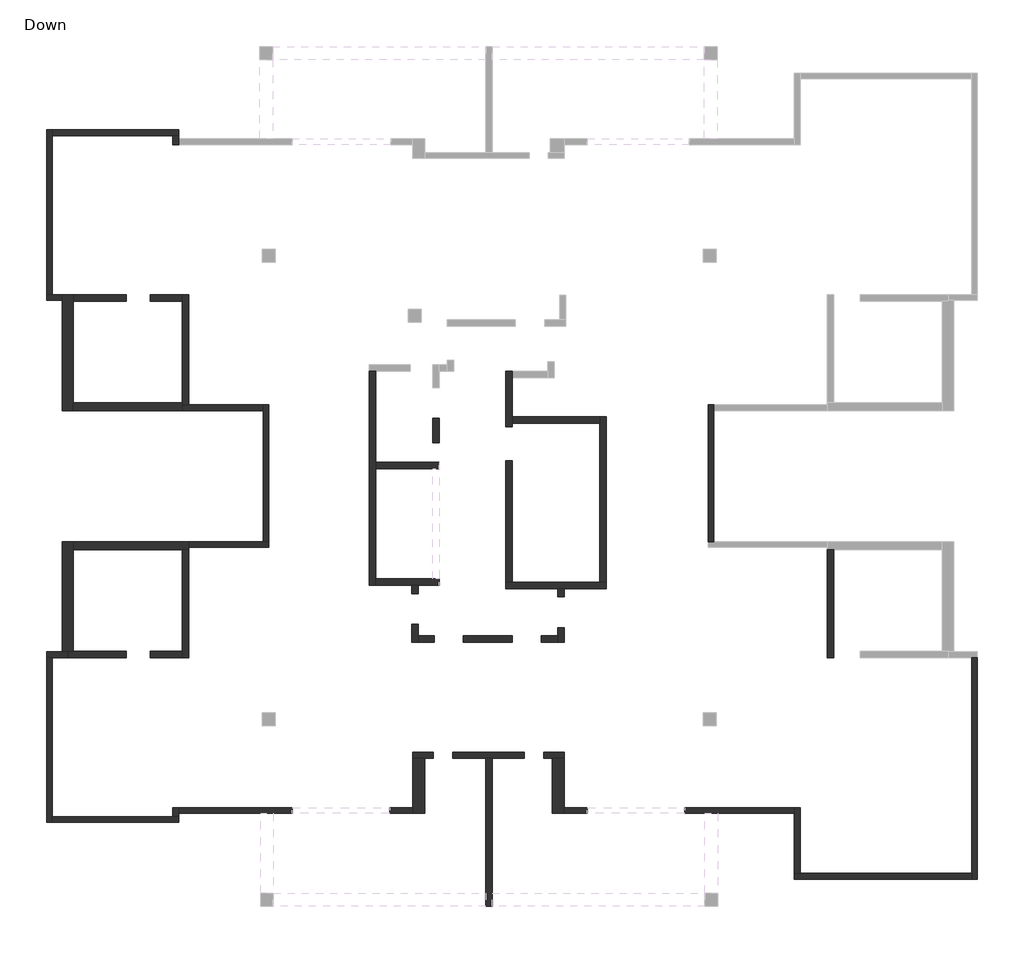
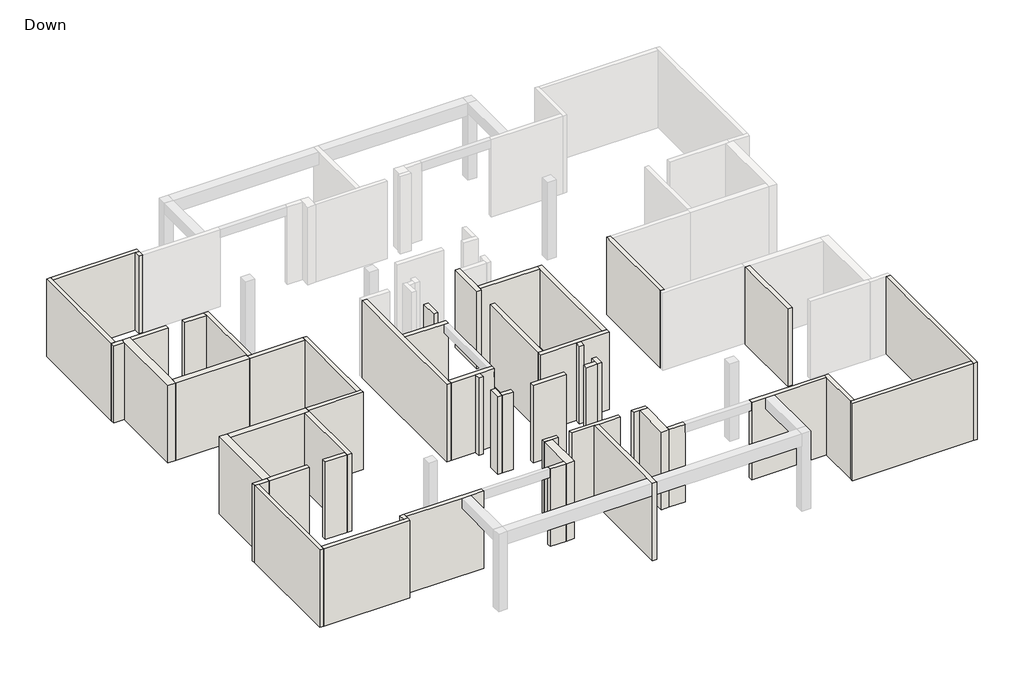
# One storey, part 1 of 2: 52 walls.
"""IFC4 building model written with IfcOpenShell, lengths in millimetres."""

from ifc_helpers import new_model, si_unit, origin, place, context, project, spatial, faceted_brep, element, save

model = new_model("IFC4")

# Units and contexts
model_context = context("Model", 3, world=origin())
ifc_project = project(units=[si_unit("LENGTHUNIT", "METRE", prefix="MILLI")], contexts=[model_context])

# Site, building, storey
site = spatial("IfcSite", under=ifc_project)
building = spatial("IfcBuilding", under=site)
storey = spatial("IfcBuildingStorey", under=building, Name="Down", Elevation=0.0)

# Walls
placement = place(None, origin())
element("IfcWall", 1, ObjectType="18", at=placement, inside=storey, context=model_context, shape_type="Brep", body=[
    faceted_brep([(-36860.6830632, 7917.598694, 0.0), (-36860.6830632, 2837.5734489, 0.0), (-36860.6830632, 2837.5734489, 3700.0), (-36860.6830632, 7917.598694, 3700.0), (-36680.6830632, 7917.598694, 0.0), (-36680.6830632, 7917.598694, 3540.0), (-36680.6830632, 7917.598694, 3700.0), (-36680.6830632, 3017.5734489, 3700.0), (-36680.6830632, 2837.5734489, 3700.0), (-36680.6830632, 2837.5734489, 0.0), (-36680.6830632, 3017.5734489, 0.0)], [[[0, 1, 2, 3]], [[4, 5, 6, 7, 8, 9, 10]], [[1, 0, 4, 10, 9]], [[3, 2, 8, 7, 6]], [[2, 1, 9, 8]], [[0, 3, 6, 5, 4]]]),
])
element("IfcWall", 2, ObjectType="18", at=placement, inside=storey, context=model_context, shape_type="Brep", body=[
    faceted_brep([(-36680.6830632, 2837.5734489, 0.0), (-32781.782199, 2837.5734489, 0.0), (-32781.782199, 2837.5734489, 3700.0), (-36680.6830632, 2837.5734489, 3700.0), (-36680.6830632, 3017.5734489, 0.0), (-36680.6830632, 3017.5734489, 3540.0), (-36680.6830632, 3017.5734489, 3700.0), (-32961.782199, 3017.5734489, 3700.0), (-32781.782199, 3017.5734489, 3700.0), (-32781.782199, 3017.5734489, 0.0), (-32961.782199, 3017.5734489, 0.0)], [[[0, 1, 2, 3]], [[4, 5, 6, 7, 8, 9, 10]], [[1, 0, 4, 10, 9]], [[3, 2, 8, 7, 6]], [[0, 3, 6, 5, 4]], [[2, 1, 9, 8]]]),
])
element("IfcWall", 3, ObjectType="18", at=placement, inside=storey, context=model_context, shape_type="Brep", body=[
    faceted_brep([(-32781.782199, 3017.5734489, 0.0), (-32781.782199, 3116.899597, 0.0), (-32781.782199, 3296.899597, 0.0), (-32781.782199, 3296.899597, 3700.0), (-32781.782199, 3116.899597, 3700.0), (-32781.782199, 3017.5734489, 3700.0), (-32961.782199, 3017.5734489, 0.0), (-32961.782199, 3017.5734489, 3540.0), (-32961.782199, 3017.5734489, 3700.0), (-32961.782199, 3296.899597, 3700.0), (-32961.782199, 3296.899597, 3540.0), (-32961.782199, 3296.899597, 0.0)], [[[0, 1, 2, 3, 4, 5]], [[6, 7, 8, 9, 10, 11]], [[2, 1, 0, 6, 11]], [[5, 4, 3, 9, 8]], [[0, 5, 8, 7, 6]], [[3, 2, 11, 10, 9]]]),
])
element("IfcWall", 4, ObjectType="18", at=placement, inside=storey, context=model_context, shape_type="Brep", body=[
    faceted_brep([(-32781.782199, 3116.899597, 0.0), (-29280.7432632, 3116.899597, 0.0), (-29280.7432632, 3116.899597, 3300.0), (-29280.7432632, 3116.899597, 3700.0), (-29861.4923547, 3116.899597, 3700.0), (-30261.4923547, 3116.899597, 3700.0), (-32781.782199, 3116.899597, 3700.0), (-32781.782199, 3296.899597, 0.0), (-32781.782199, 3296.899597, 3700.0), (-29280.7432632, 3296.899597, 3700.0), (-29280.7432632, 3296.899597, 3300.0), (-29280.7432632, 3296.899597, 0.0)], [[[0, 1, 2, 3, 4, 5, 6]], [[7, 8, 9, 10, 11]], [[1, 0, 7, 11]], [[3, 2, 1, 11, 10, 9]], [[6, 5, 4, 3, 9, 8]], [[0, 6, 8, 7]]]),
])
element("IfcWall", 5, ObjectType="18", at=placement, inside=storey, context=model_context, shape_type="Brep", body=[
    faceted_brep([(-26281.3646827, 3116.899597, 0.0), (-25559.7256887, 3116.899597, 0.0), (-25559.7256887, 3116.899597, 3700.0), (-26281.3646827, 3116.899597, 3700.0), (-26281.3646827, 3116.899597, 3300.0), (-26281.3646827, 3296.899597, 0.0), (-26281.3646827, 3296.899597, 3300.0), (-26281.3646827, 3296.899597, 3700.0), (-25559.7256887, 3296.899597, 3700.0), (-25559.7256887, 3296.899597, 3540.0), (-25559.7256887, 3296.899597, 0.0)], [[[0, 1, 2, 3, 4]], [[5, 6, 7, 8, 9, 10]], [[1, 0, 5, 10]], [[3, 2, 8, 7]], [[0, 4, 3, 7, 6, 5]], [[2, 1, 10, 9, 8]]]),
])
element("IfcWall", 6, ObjectType="18", at=placement, inside=storey, context=model_context, shape_type="Brep", body=[
    faceted_brep([(-25559.7256887, 4816.6180163, 0.0), (-25199.7256887, 4816.6180163, 0.0), (-24930.9034729, 4816.6180163, 0.0), (-24930.9034729, 4816.6180163, 3540.0), (-24930.9034729, 4816.6180163, 3700.0), (-25199.7256887, 4816.6180163, 3700.0), (-25559.7256887, 4816.6180163, 3700.0), (-25559.7256887, 4996.6180163, 0.0), (-25559.7256887, 4996.6180163, 3540.0), (-25559.7256887, 4996.6180163, 3700.0), (-24930.9034729, 4996.6180163, 3700.0), (-24930.9034729, 4996.6180163, 3540.0), (-24930.9034729, 4996.6180163, 0.0)], [[[0, 1, 2, 3, 4, 5, 6]], [[7, 8, 9, 10, 11, 12]], [[2, 1, 0, 7, 12]], [[4, 3, 2, 12, 11, 10]], [[6, 5, 4, 10, 9]], [[0, 6, 9, 8, 7]]]),
])
element("IfcWall", 7, ObjectType="18", at=placement, inside=storey, context=model_context, shape_type="Brep", body=[
    faceted_brep([(-24329.7577306, 4816.6180163, 0.0), (-23311.6200473, 4816.6180163, 0.0), (-23111.6200473, 4816.6180163, 0.0), (-22130.4956663, 4816.6180163, 0.0), (-22130.4956663, 4816.6180163, 3540.0), (-22130.4956663, 4816.6180163, 3700.0), (-23111.6200473, 4816.6180163, 3700.0), (-23311.6200473, 4816.6180163, 3700.0), (-24329.7577306, 4816.6180163, 3700.0), (-24329.7577306, 4816.6180163, 3540.0), (-24329.7577306, 4996.6180163, 0.0), (-24329.7577306, 4996.6180163, 3540.0), (-24329.7577306, 4996.6180163, 3700.0), (-22130.4956663, 4996.6180163, 3700.0), (-22130.4956663, 4996.6180163, 3540.0), (-22130.4956663, 4996.6180163, 0.0)], [[[0, 1, 2, 3, 4, 5, 6, 7, 8, 9]], [[10, 11, 12, 13, 14, 15]], [[3, 2, 1, 0, 10, 15]], [[5, 4, 3, 15, 14, 13]], [[8, 7, 6, 5, 13, 12]], [[0, 9, 8, 12, 11, 10]]]),
])
element("IfcWall", 8, ObjectType="18", at=placement, inside=storey, context=model_context, shape_type="Brep", body=[
    faceted_brep([(-36860.6830632, 7917.598694, 0.0), (-36680.6830632, 7917.598694, 0.0), (-36205.9326019, 7917.598694, 0.0), (-36205.9326019, 7917.598694, 3540.0), (-36205.9326019, 7917.598694, 3700.0), (-36680.6830632, 7917.598694, 3700.0), (-36860.6830632, 7917.598694, 3700.0), (-36860.6830632, 8097.598694, 0.0), (-36860.6830632, 8097.598694, 3700.0), (-36380.9326019, 8097.598694, 3700.0), (-36205.9326019, 8097.598694, 3700.0), (-36205.9326019, 8097.598694, 0.0), (-36380.9326019, 8097.598694, 0.0)], [[[0, 1, 2, 3, 4, 5, 6]], [[7, 8, 9, 10, 11, 12]], [[2, 1, 0, 7, 12, 11]], [[4, 3, 2, 11, 10]], [[6, 5, 4, 10, 9, 8]], [[0, 6, 8, 7]]]),
])
element("IfcWall", 9, ObjectType="18", at=placement, inside=storey, context=model_context, shape_type="Brep", body=[
    faceted_brep([(-32480.1801017, 11317.0355326, 0.0), (-30000.4247857, 11317.0355326, 0.0), (-30000.4247857, 11317.0355326, 3540.0), (-30000.4247857, 11317.0355326, 3700.0), (-32480.1801017, 11317.0355326, 3700.0), (-32480.1801017, 11317.0355326, 3540.0), (-32480.1801017, 11497.0355326, 0.0), (-32480.1801017, 11497.0355326, 3700.0), (-30180.4247857, 11497.0355326, 3700.0), (-30000.4247857, 11497.0355326, 3700.0), (-30000.4247857, 11497.0355326, 0.0), (-30180.4247857, 11497.0355326, 0.0)], [[[0, 1, 2, 3, 4, 5]], [[6, 7, 8, 9, 10, 11]], [[1, 0, 6, 11, 10]], [[4, 3, 9, 8, 7]], [[0, 5, 4, 7, 6]], [[3, 2, 1, 10, 9]]]),
])
element("IfcWall", 10, ObjectType="18", at=placement, inside=storey, context=model_context, shape_type="Brep", body=[
    faceted_brep([(-30000.4247857, 11497.0355326, 0.0), (-30000.4247857, 15717.7559909, 0.0), (-30000.4247857, 15717.7559909, 3540.0), (-30000.4247857, 15717.7559909, 3700.0), (-30000.4247857, 13517.3957617, 3700.0), (-30000.4247857, 11497.0355326, 3700.0), (-30180.4247857, 11497.0355326, 0.0), (-30180.4247857, 11497.0355326, 3700.0), (-30180.4247857, 15537.7559909, 3700.0), (-30180.4247857, 15717.7559909, 3700.0), (-30180.4247857, 15717.7559909, 0.0), (-30180.4247857, 15537.7559909, 0.0)], [[[0, 1, 2, 3, 4, 5]], [[6, 7, 8, 9, 10, 11]], [[1, 0, 6, 11, 10]], [[5, 4, 3, 9, 8, 7]], [[0, 5, 7, 6]], [[3, 2, 1, 10, 9]]]),
])
element("IfcWall", 11, ObjectType="18", at=placement, inside=storey, context=model_context, shape_type="Brep", body=[
    faceted_brep([(-8329.623737, 7917.598694, 0.0), (-8329.623737, 1267.053981, 0.0), (-8329.623737, 1087.053981, 0.0), (-8329.623737, 1087.053981, 3700.0), (-8329.623737, 1267.053981, 3700.0), (-8329.623737, 7917.598694, 3700.0), (-8329.623737, 7917.598694, 3540.0), (-8149.623737, 7917.598694, 0.0), (-8149.623737, 7917.598694, 3700.0), (-8149.623737, 1087.053981, 3700.0), (-8149.623737, 1087.053981, 0.0)], [[[0, 1, 2, 3, 4, 5, 6]], [[7, 8, 9, 10]], [[2, 1, 0, 7, 10]], [[5, 4, 3, 9, 8]], [[3, 2, 10, 9]], [[0, 6, 5, 8, 7]]]),
])
element("IfcWall", 12, ObjectType="18", at=placement, inside=storey, context=model_context, shape_type="Brep", body=[
    faceted_brep([(-8329.623737, 1267.053981, 0.0), (-13621.2403988, 1267.053981, 0.0), (-13801.2403988, 1267.053981, 0.0), (-13801.2403988, 1267.053981, 3700.0), (-13621.2403988, 1267.053981, 3700.0), (-8329.623737, 1267.053981, 3700.0), (-8329.623737, 1267.053981, 3540.0), (-8329.623737, 1087.053981, 0.0), (-8329.623737, 1087.053981, 3700.0), (-13801.2403988, 1087.053981, 3700.0), (-13801.2403988, 1087.053981, 0.0)], [[[0, 1, 2, 3, 4, 5, 6]], [[7, 8, 9, 10]], [[2, 1, 0, 7, 10]], [[5, 4, 3, 9, 8]], [[0, 6, 5, 8, 7]], [[3, 2, 10, 9]]]),
])
element("IfcWall", 13, ObjectType="18", at=placement, inside=storey, context=model_context, shape_type="Brep", body=[
    faceted_brep([(-13621.2403988, 1267.053981, 0.0), (-13621.2403988, 3296.899597, 0.0), (-13621.2403988, 3296.899597, 3540.0), (-13621.2403988, 3296.899597, 3700.0), (-13621.2403988, 1267.053981, 3700.0), (-13621.2403988, 1267.053981, 3540.0), (-13801.2403988, 1267.053981, 0.0), (-13801.2403988, 1267.053981, 3700.0), (-13801.2403988, 3116.899597, 3700.0), (-13801.2403988, 3296.899597, 3700.0), (-13801.2403988, 3296.899597, 0.0), (-13801.2403988, 3116.899597, 0.0)], [[[0, 1, 2, 3, 4, 5]], [[6, 7, 8, 9, 10, 11]], [[1, 0, 6, 11, 10]], [[4, 3, 9, 8, 7]], [[0, 5, 4, 7, 6]], [[3, 2, 1, 10, 9]]]),
])
element("IfcWall", 14, ObjectType="18", at=placement, inside=storey, context=model_context, shape_type="Brep", body=[
    faceted_brep([(-13801.2403988, 3296.899597, 0.0), (-17179.5101337, 3296.899597, 0.0), (-17179.5101337, 3296.899597, 3300.0), (-17179.5101337, 3296.899597, 3700.0), (-13801.2403988, 3296.899597, 3700.0), (-13801.2403988, 3116.899597, 0.0), (-13801.2403988, 3116.899597, 3700.0), (-16161.2977307, 3116.899597, 3700.0), (-16561.2977307, 3116.899597, 3700.0), (-17179.5101337, 3116.899597, 3700.0), (-17179.5101337, 3116.899597, 3300.0), (-17179.5101337, 3116.899597, 0.0)], [[[0, 1, 2, 3, 4]], [[5, 6, 7, 8, 9, 10, 11]], [[1, 0, 5, 11]], [[3, 2, 1, 11, 10, 9]], [[4, 3, 9, 8, 7, 6]], [[0, 4, 6, 5]]]),
])
element("IfcWall", 15, ObjectType="18", at=placement, inside=storey, context=model_context, shape_type="Brep", body=[
    faceted_brep([(-20181.0054246, 3296.899597, 0.0), (-20900.5277083, 3296.899597, 0.0), (-20900.5277083, 3296.899597, 3540.0), (-20900.5277083, 3296.899597, 3700.0), (-20181.0054246, 3296.899597, 3700.0), (-20181.0054246, 3296.899597, 3300.0), (-20181.0054246, 3116.899597, 0.0), (-20181.0054246, 3116.899597, 3300.0), (-20181.0054246, 3116.899597, 3700.0), (-20900.5277083, 3116.899597, 3700.0), (-20900.5277083, 3116.899597, 0.0)], [[[0, 1, 2, 3, 4, 5]], [[6, 7, 8, 9, 10]], [[1, 0, 6, 10]], [[4, 3, 9, 8]], [[0, 5, 4, 8, 7, 6]], [[3, 2, 1, 10, 9]]]),
])
element("IfcWall", 16, ObjectType="18", at=placement, inside=storey, context=model_context, shape_type="Brep", body=[
    faceted_brep([(-20900.5277083, 4996.6180163, 0.0), (-21531.4666344, 4996.6180163, 0.0), (-21531.4666344, 4996.6180163, 3540.0), (-21531.4666344, 4996.6180163, 3700.0), (-20900.5277083, 4996.6180163, 3700.0), (-20900.5277083, 4996.6180163, 3540.0), (-20900.5277083, 4816.6180163, 0.0), (-20900.5277083, 4816.6180163, 3700.0), (-21260.5277083, 4816.6180163, 3700.0), (-21531.4666344, 4816.6180163, 3700.0), (-21531.4666344, 4816.6180163, 3540.0), (-21531.4666344, 4816.6180163, 0.0), (-21260.5277083, 4816.6180163, 0.0)], [[[0, 1, 2, 3, 4, 5]], [[6, 7, 8, 9, 10, 11, 12]], [[1, 0, 6, 12, 11]], [[3, 2, 1, 11, 10, 9]], [[4, 3, 9, 8, 7]], [[0, 5, 4, 7, 6]]]),
])
element("IfcWall", 17, ObjectType="18", at=placement, inside=storey, context=model_context, shape_type="Brep", body=[
    faceted_brep([(-16279.8286113, 11497.0355326, 0.0), (-16279.8286113, 15537.7559909, 0.0), (-16279.8286113, 15717.7559909, 0.0), (-16279.8286113, 15717.7559909, 3700.0), (-16279.8286113, 15537.7559909, 3700.0), (-16279.8286113, 11497.0355326, 3700.0), (-16459.8286113, 11497.0355326, 0.0), (-16459.8286113, 11497.0355326, 3700.0), (-16459.8286113, 15347.3316778, 3700.0), (-16459.8286113, 15717.7559909, 3700.0), (-16459.8286113, 15717.7559909, 3540.0), (-16459.8286113, 15717.7559909, 0.0)], [[[0, 1, 2, 3, 4, 5]], [[6, 7, 8, 9, 10, 11]], [[2, 1, 0, 6, 11]], [[5, 4, 3, 9, 8, 7]], [[0, 5, 7, 6]], [[3, 2, 11, 10, 9]]]),
])
element("IfcWall", 18, ObjectType="18", at=placement, inside=storey, context=model_context, shape_type="Brep", body=[
    faceted_brep([(-30180.4247857, 15717.7559909, 0.0), (-32481.2093278, 15717.7559909, 0.0), (-32681.2093278, 15717.7559909, 0.0), (-32681.2093278, 15717.7559909, 3700.0), (-32481.2093278, 15717.7559909, 3700.0), (-30180.4247857, 15717.7559909, 3700.0), (-30180.4247857, 15537.7559909, 0.0), (-30180.4247857, 15537.7559909, 3700.0), (-32681.2093278, 15537.7559909, 3700.0), (-32681.2093278, 15537.7559909, 0.0)], [[[0, 1, 2, 3, 4, 5]], [[6, 7, 8, 9]], [[2, 1, 0, 6, 9]], [[5, 4, 3, 8, 7]], [[0, 5, 7, 6]], [[3, 2, 9, 8]]]),
])
element("IfcWall", 19, ObjectType="18", at=placement, inside=storey, context=model_context, shape_type="Brep", body=[
    faceted_brep([(-36380.1898114, 19117.1928294, 0.0), (-36680.6830632, 19117.1928294, 0.0), (-36860.6830632, 19117.1928294, 0.0), (-36860.6830632, 19117.1928294, 3700.0), (-36680.6830632, 19117.1928294, 3700.0), (-36380.1898114, 19117.1928294, 3700.0), (-36380.1898114, 18937.1928294, 0.0), (-36380.1898114, 18937.1928294, 3700.0), (-36860.6830632, 18937.1928294, 3700.0), (-36860.6830632, 18937.1928294, 0.0)], [[[0, 1, 2, 3, 4, 5]], [[6, 7, 8, 9]], [[2, 1, 0, 6, 9]], [[5, 4, 3, 8, 7]], [[3, 2, 9, 8]], [[0, 5, 7, 6]]]),
])
element("IfcWall", 20, ObjectType="18", at=placement, inside=storey, context=model_context, shape_type="Brep", body=[
    faceted_brep([(-36680.6830632, 19117.1928294, 0.0), (-36680.6830632, 24017.2976939, 0.0), (-36680.6830632, 24197.2976939, 0.0), (-36680.6830632, 24197.2976939, 3700.0), (-36680.6830632, 24017.2976939, 3700.0), (-36680.6830632, 19117.1928294, 3700.0), (-36680.6830632, 19117.1928294, 3540.0), (-36860.6830632, 19117.1928294, 0.0), (-36860.6830632, 19117.1928294, 3700.0), (-36860.6830632, 24197.2976939, 3700.0), (-36860.6830632, 24197.2976939, 0.0)], [[[0, 1, 2, 3, 4, 5, 6]], [[7, 8, 9, 10]], [[2, 1, 0, 7, 10]], [[5, 4, 3, 9, 8]], [[0, 6, 5, 8, 7]], [[3, 2, 10, 9]]]),
])
element("IfcWall", 21, ObjectType="18", at=placement, inside=storey, context=model_context, shape_type="Brep", body=[
    faceted_brep([(-36680.6830632, 24017.2976939, 0.0), (-32961.782199, 24017.2976939, 0.0), (-32781.782199, 24017.2976939, 0.0), (-32781.782199, 24017.2976939, 3700.0), (-32961.782199, 24017.2976939, 3700.0), (-36680.6830632, 24017.2976939, 3700.0), (-36680.6830632, 24017.2976939, 3540.0), (-36680.6830632, 24197.2976939, 0.0), (-36680.6830632, 24197.2976939, 3700.0), (-32781.782199, 24197.2976939, 3700.0), (-32781.782199, 24197.2976939, 0.0)], [[[0, 1, 2, 3, 4, 5, 6]], [[7, 8, 9, 10]], [[2, 1, 0, 7, 10]], [[5, 4, 3, 9, 8]], [[0, 6, 5, 8, 7]], [[3, 2, 10, 9]]]),
])
element("IfcWall", 22, ObjectType="18", at=placement, inside=storey, context=model_context, shape_type="Brep", body=[
    faceted_brep([(-32961.782199, 24017.2976939, 0.0), (-32961.782199, 23737.9715458, 0.0), (-32961.782199, 23737.9715458, 3540.0), (-32961.782199, 23737.9715458, 3700.0), (-32961.782199, 24017.2976939, 3700.0), (-32961.782199, 24017.2976939, 3540.0), (-32781.782199, 24017.2976939, 0.0), (-32781.782199, 24017.2976939, 3700.0), (-32781.782199, 23917.9715458, 3700.0), (-32781.782199, 23737.9715458, 3700.0), (-32781.782199, 23737.9715458, 0.0), (-32781.782199, 23917.9715458, 0.0)], [[[0, 1, 2, 3, 4, 5]], [[6, 7, 8, 9, 10, 11]], [[1, 0, 6, 11, 10]], [[4, 3, 9, 8, 7]], [[0, 5, 4, 7, 6]], [[3, 2, 1, 10, 9]]]),
])
element("IfcWall", 23, ObjectType="20", at=placement, inside=storey, context=model_context, shape_type="Brep", body=[
    faceted_brep([(-34401.0656246, 8116.6490873, 0.0), (-36030.9326019, 8116.6490873, 0.0), (-36205.9326019, 8116.6490873, 0.0), (-36205.9326019, 8116.6490873, 3700.0), (-36030.9326019, 8116.6490873, 3700.0), (-34401.0656246, 8116.6490873, 3700.0), (-34401.0656246, 8116.6490873, 3540.0), (-34401.0656246, 7916.6490873, 0.0), (-34401.0656246, 7916.6490873, 3540.0), (-34401.0656246, 7916.6490873, 3700.0), (-36205.9326019, 7916.6490873, 3700.0), (-36205.9326019, 7916.6490873, 3540.0), (-36205.9326019, 7916.6490873, 0.0), (-36205.9326019, 7917.598694, 0.0), (-36205.9326019, 8097.598694, 0.0), (-36205.9326019, 7917.598694, 3700.0), (-36205.9326019, 8097.598694, 3700.0), (-34401.0656246, 8111.6490873, 3700.0)], [[[0, 1, 2, 3, 4, 5, 6]], [[7, 8, 9, 10, 11, 12]], [[2, 1, 0, 7, 12, 13, 14]], [[3, 2, 14, 13, 12, 11, 10, 15, 16]], [[5, 4, 3, 16, 15, 10, 9, 17]], [[0, 6, 5, 17, 9, 8, 7]]]),
])
element("IfcWall", 24, ObjectType="20", at=placement, inside=storey, context=model_context, shape_type="Brep", body=[
    faceted_brep([(-32680.1801017, 11247.0355326, 0.0), (-32680.1801017, 8117.6783134, 0.0), (-32680.1801017, 7917.6783134, 0.0), (-32680.1801017, 7917.6783134, 3700.0), (-32680.1801017, 8117.6783134, 3700.0), (-32680.1801017, 11247.0355326, 3700.0), (-32680.1801017, 11247.0355326, 3540.0), (-32480.1801017, 11247.0355326, 0.0), (-32480.1801017, 11247.0355326, 3700.0), (-32480.1801017, 7917.6783134, 3700.0), (-32480.1801017, 7917.6783134, 3540.0), (-32480.1801017, 7917.6783134, 0.0)], [[[0, 1, 2, 3, 4, 5, 6]], [[7, 8, 9, 10, 11]], [[2, 1, 0, 7, 11]], [[5, 4, 3, 9, 8]], [[0, 6, 5, 8, 7]], [[3, 2, 11, 10, 9]]]),
])
element("IfcWall", 25, ObjectType="20", at=placement, inside=storey, context=model_context, shape_type="Brep", body=[
    faceted_brep([(-32680.1801017, 8117.6783134, 0.0), (-33660.2169985, 8117.6783134, 0.0), (-33660.2169985, 8117.6783134, 3540.0), (-33660.2169985, 8117.6783134, 3700.0), (-32680.1801017, 8117.6783134, 3700.0), (-32680.1801017, 8117.6783134, 3540.0), (-32680.1801017, 7917.6783134, 0.0), (-32680.1801017, 7917.6783134, 3700.0), (-33660.2169985, 7917.6783134, 3700.0), (-33660.2169985, 7917.6783134, 3540.0), (-33660.2169985, 7917.6783134, 0.0), (-33660.2169985, 8111.6490873, 3700.0)], [[[0, 1, 2, 3, 4, 5]], [[6, 7, 8, 9, 10]], [[1, 0, 6, 10]], [[3, 2, 1, 10, 9, 8, 11]], [[4, 3, 11, 8, 7]], [[0, 5, 4, 7, 6]]]),
])
element("IfcWall", 26, ObjectType="20", at=placement, inside=storey, context=model_context, shape_type="Brep", body=[
    faceted_brep([(-23311.6200473, 4816.6180163, 0.0), (-23311.6200473, 259.7166846, 0.0), (-23311.6200473, 259.7166846, 3100.0), (-23311.6200473, 259.7166846, 3700.0), (-23311.6200473, 659.7166846, 3700.0), (-23311.6200473, 4816.6180163, 3700.0), (-23311.6200473, 4816.6180163, 3540.0), (-23111.6200473, 4816.6180163, 0.0), (-23111.6200473, 4816.6180163, 3540.0), (-23111.6200473, 4816.6180163, 3700.0), (-23111.6200473, 659.7166846, 3700.0), (-23111.6200473, 259.7166846, 3700.0), (-23111.6200473, 259.7166846, 3100.0), (-23111.6200473, 259.7166846, 0.0)], [[[0, 1, 2, 3, 4, 5, 6]], [[7, 8, 9, 10, 11, 12, 13]], [[1, 0, 7, 13]], [[3, 2, 1, 13, 12, 11]], [[5, 4, 3, 11, 10, 9]], [[0, 6, 5, 9, 8, 7]]]),
])
element("IfcWall", 27, ObjectType="20", at=placement, inside=storey, context=model_context, shape_type="Brep", body=[
    faceted_brep([(-12779.898521, 11247.0355326, 0.0), (-12779.898521, 7917.6783134, 0.0), (-12779.898521, 7917.6783134, 3540.0), (-12779.898521, 7917.6783134, 3700.0), (-12779.898521, 11247.0355326, 3700.0), (-12579.898521, 11247.0355326, 0.0), (-12579.898521, 11247.0355326, 3540.0), (-12579.898521, 11247.0355326, 3700.0), (-12579.898521, 8116.6490873, 3700.0), (-12579.898521, 7917.6783134, 3700.0), (-12579.898521, 7917.6783134, 3540.0), (-12579.898521, 7917.6783134, 0.0)], [[[0, 1, 2, 3, 4]], [[5, 6, 7, 8, 9, 10, 11]], [[1, 0, 5, 11]], [[3, 2, 1, 11, 10, 9]], [[4, 3, 9, 8, 7]], [[0, 4, 7, 6, 5]]]),
])
element("IfcWall", 28, ObjectType="20", at=placement, inside=storey, context=model_context, shape_type="Brep", body=[
    faceted_brep([(-32481.2093278, 15717.7559909, 0.0), (-32481.2093278, 19117.1928294, 0.0), (-32481.2093278, 19117.1928294, 3540.0), (-32481.2093278, 19117.1928294, 3700.0), (-32481.2093278, 15717.7559909, 3700.0), (-32481.2093278, 15717.7559909, 3540.0), (-32681.2093278, 15717.7559909, 0.0), (-32681.2093278, 15717.7559909, 3700.0), (-32681.2093278, 15787.8356102, 3700.0), (-32681.2093278, 18917.1928294, 3700.0), (-32681.2093278, 19117.1928294, 3700.0), (-32681.2093278, 19117.1928294, 0.0), (-32681.2093278, 18917.1928294, 0.0), (-32681.2093278, 15787.8356102, 0.0)], [[[0, 1, 2, 3, 4, 5]], [[6, 7, 8, 9, 10, 11, 12, 13]], [[1, 0, 6, 13, 12, 11]], [[4, 3, 10, 9, 8, 7]], [[0, 5, 4, 7, 6]], [[3, 2, 1, 11, 10]]]),
])
element("IfcWall", 29, ObjectType="20", at=placement, inside=storey, context=model_context, shape_type="Brep", body=[
    faceted_brep([(-32681.2093278, 19117.1928294, 0.0), (-33660.2169985, 19117.1928294, 0.0), (-33660.2169985, 19117.1928294, 3540.0), (-33660.2169985, 19117.1928294, 3700.0), (-32681.2093278, 19117.1928294, 3700.0), (-32681.2093278, 18917.1928294, 0.0), (-32681.2093278, 18917.1928294, 3540.0), (-32681.2093278, 18917.1928294, 3700.0), (-33660.2169985, 18917.1928294, 3700.0), (-33660.2169985, 18917.1928294, 3540.0), (-33660.2169985, 18917.1928294, 0.0)], [[[0, 1, 2, 3, 4]], [[5, 6, 7, 8, 9, 10]], [[1, 0, 5, 10]], [[3, 2, 1, 10, 9, 8]], [[4, 3, 8, 7]], [[0, 4, 7, 6, 5]]]),
])
element("IfcWall", 30, ObjectType="20", at=placement, inside=storey, context=model_context, shape_type="Brep", body=[
    faceted_brep([(-34401.0656246, 19117.1928294, 0.0), (-36030.1898114, 19117.1928294, 0.0), (-36030.1898114, 19117.1928294, 3700.0), (-34401.0656246, 19117.1928294, 3700.0), (-34401.0656246, 19117.1928294, 3540.0), (-34401.0656246, 18917.1928294, 0.0), (-34401.0656246, 18917.1928294, 3540.0), (-34401.0656246, 18917.1928294, 3700.0), (-36030.1898114, 18917.1928294, 3700.0), (-36030.1898114, 18917.1928294, 3540.0), (-36030.1898114, 18917.1928294, 0.0)], [[[0, 1, 2, 3, 4]], [[5, 6, 7, 8, 9, 10]], [[1, 0, 5, 10]], [[3, 2, 8, 7]], [[0, 4, 3, 7, 6, 5]], [[2, 1, 10, 9, 8]]]),
])
element("IfcWall", 31, ObjectType="20", at=placement, inside=storey, context=model_context, shape_type="Brep", body=[
    faceted_brep([(-25399.7839467, 9896.8025002, 0.0), (-25399.7839467, 10146.5743227, 0.0), (-25399.7839467, 10146.5743227, 3540.0), (-25399.7839467, 10146.5743227, 3700.0), (-25399.7839467, 9896.8025002, 3700.0), (-25399.7839467, 9896.8025002, 3540.0), (-25599.7839467, 9896.8025002, 0.0), (-25599.7839467, 9896.8025002, 3540.0), (-25599.7839467, 9896.8025002, 3700.0), (-25599.7839467, 10146.5743227, 3700.0), (-25599.7839467, 10146.5743227, 3540.0), (-25599.7839467, 10146.5743227, 0.0)], [[[0, 1, 2, 3, 4, 5]], [[6, 7, 8, 9, 10, 11]], [[1, 0, 6, 11]], [[4, 3, 9, 8]], [[0, 5, 4, 8, 7, 6]], [[3, 2, 1, 11, 10, 9]]]),
])
element("IfcWall", 32, ObjectType="20", at=placement, inside=storey, context=model_context, shape_type="Brep", body=[
    faceted_brep([(-25599.7839467, 8946.3995485, 0.0), (-25599.7839467, 8396.0548548, 0.0), (-25599.7839467, 8396.0548548, 3540.0), (-25599.7839467, 8396.0548548, 3700.0), (-25599.7839467, 8946.3995485, 3700.0), (-25599.7839467, 8946.3995485, 3540.0), (-25399.7839467, 8946.3995485, 0.0), (-25399.7839467, 8946.3995485, 3540.0), (-25399.7839467, 8946.3995485, 3700.0), (-25399.7839467, 8596.0548548, 3700.0), (-25399.7839467, 8396.0548548, 3700.0), (-25399.7839467, 8396.0548548, 0.0), (-25399.7839467, 8596.0548548, 0.0)], [[[0, 1, 2, 3, 4, 5]], [[6, 7, 8, 9, 10, 11, 12]], [[1, 0, 6, 12, 11]], [[4, 3, 10, 9, 8]], [[0, 5, 4, 8, 7, 6]], [[3, 2, 1, 11, 10]]]),
])
element("IfcWall", 33, ObjectType="20", at=placement, inside=storey, context=model_context, shape_type="Brep", body=[
    faceted_brep([(-25399.7839467, 8396.0548548, 0.0), (-24901.2695279, 8396.0548548, 0.0), (-24901.2695279, 8396.0548548, 3540.0), (-24901.2695279, 8396.0548548, 3700.0), (-25399.7839467, 8396.0548548, 3700.0), (-25399.7839467, 8596.0548548, 0.0), (-25399.7839467, 8596.0548548, 3540.0), (-25399.7839467, 8596.0548548, 3700.0), (-24901.2695279, 8596.0548548, 3700.0), (-24901.2695279, 8596.0548548, 3540.0), (-24901.2695279, 8596.0548548, 0.0)], [[[0, 1, 2, 3, 4]], [[5, 6, 7, 8, 9, 10]], [[1, 0, 5, 10]], [[3, 2, 1, 10, 9, 8]], [[4, 3, 8, 7]], [[0, 4, 7, 6, 5]]]),
])
element("IfcWall", 34, ObjectType="20", at=placement, inside=storey, context=model_context, shape_type="Brep", body=[
    faceted_brep([(-24001.6676248, 8396.0548548, 0.0), (-22500.9199794, 8396.0548548, 0.0), (-22500.9199794, 8396.0548548, 3540.0), (-22500.9199794, 8396.0548548, 3700.0), (-24001.6676248, 8396.0548548, 3700.0), (-24001.6676248, 8396.0548548, 3540.0), (-24001.6676248, 8596.0548548, 0.0), (-24001.6676248, 8596.0548548, 3540.0), (-24001.6676248, 8596.0548548, 3700.0), (-22500.9199794, 8596.0548548, 3700.0), (-22500.9199794, 8596.0548548, 3540.0), (-22500.9199794, 8596.0548548, 0.0)], [[[0, 1, 2, 3, 4, 5]], [[6, 7, 8, 9, 10, 11]], [[1, 0, 6, 11]], [[3, 2, 1, 11, 10, 9]], [[4, 3, 9, 8]], [[0, 5, 4, 8, 7, 6]]]),
])
element("IfcWall", 35, ObjectType="20", at=placement, inside=storey, context=model_context, shape_type="Brep", body=[
    faceted_brep([(-21601.3180763, 8396.0548548, 0.0), (-21100.686947, 8396.0548548, 0.0), (-21100.686947, 8396.0548548, 3700.0), (-21601.3180763, 8396.0548548, 3700.0), (-21601.3180763, 8396.0548548, 3540.0), (-21601.3180763, 8596.0548548, 0.0), (-21601.3180763, 8596.0548548, 3540.0), (-21601.3180763, 8596.0548548, 3700.0), (-21100.686947, 8596.0548548, 3700.0), (-21100.686947, 8596.0548548, 3540.0), (-21100.686947, 8596.0548548, 0.0)], [[[0, 1, 2, 3, 4]], [[5, 6, 7, 8, 9, 10]], [[1, 0, 5, 10]], [[3, 2, 8, 7]], [[0, 4, 3, 7, 6, 5]], [[2, 1, 10, 9, 8]]]),
])
element("IfcWall", 36, ObjectType="20", at=placement, inside=storey, context=model_context, shape_type="Brep", body=[
    faceted_brep([(-20900.686947, 8396.0548548, 0.0), (-20900.686947, 8846.9141616, 0.0), (-20900.686947, 8846.9141616, 3540.0), (-20900.686947, 8846.9141616, 3700.0), (-20900.686947, 8396.0548548, 3700.0), (-20900.686947, 8396.0548548, 3540.0), (-21100.686947, 8396.0548548, 0.0), (-21100.686947, 8396.0548548, 3700.0), (-21100.686947, 8596.0548548, 3700.0), (-21100.686947, 8846.9141616, 3700.0), (-21100.686947, 8846.9141616, 3540.0), (-21100.686947, 8846.9141616, 0.0), (-21100.686947, 8596.0548548, 0.0)], [[[0, 1, 2, 3, 4, 5]], [[6, 7, 8, 9, 10, 11, 12]], [[1, 0, 6, 12, 11]], [[3, 2, 1, 11, 10, 9]], [[4, 3, 9, 8, 7]], [[0, 5, 4, 7, 6]]]),
])
element("IfcWall", 37, ObjectType="20", at=placement, inside=storey, context=model_context, shape_type="Brep", body=[
    faceted_brep([(-20900.686947, 9797.3171133, 0.0), (-20900.686947, 10047.0889358, 0.0), (-20900.686947, 10047.0889358, 3540.0), (-20900.686947, 10047.0889358, 3700.0), (-20900.686947, 9797.3171133, 3700.0), (-20900.686947, 9797.3171133, 3540.0), (-21100.686947, 9797.3171133, 0.0), (-21100.686947, 9797.3171133, 3540.0), (-21100.686947, 9797.3171133, 3700.0), (-21100.686947, 10047.0889358, 3700.0), (-21100.686947, 10047.0889358, 3540.0), (-21100.686947, 10047.0889358, 0.0)], [[[0, 1, 2, 3, 4, 5]], [[6, 7, 8, 9, 10, 11]], [[1, 0, 6, 11]], [[4, 3, 9, 8]], [[0, 5, 4, 8, 7, 6]], [[3, 2, 1, 11, 10, 9]]]),
])
element("IfcWall", 38, ObjectType="20", at=placement, inside=storey, context=model_context, shape_type="Brep", body=[
    faceted_brep([(-19601.0267859, 10247.0889358, 0.0), (-19801.0267859, 10247.0889358, 0.0), (-22499.8907532, 10247.0889358, 0.0), (-22699.8907532, 10247.0889358, 0.0), (-22699.8907532, 10247.0889358, 3700.0), (-22499.8907532, 10247.0889358, 3700.0), (-19801.0267859, 10247.0889358, 3700.0), (-19601.0267859, 10247.0889358, 3700.0), (-19601.0267859, 10047.0889358, 0.0), (-19601.0267859, 10047.0889358, 3540.0), (-19601.0267859, 10047.0889358, 3700.0), (-20900.686947, 10047.0889358, 3700.0), (-21100.686947, 10047.0889358, 3700.0), (-22699.8907532, 10047.0889358, 3700.0), (-22699.8907532, 10047.0889358, 3540.0), (-22699.8907532, 10047.0889358, 0.0), (-21100.686947, 10047.0889358, 0.0), (-20900.686947, 10047.0889358, 0.0)], [[[0, 1, 2, 3, 4, 5, 6, 7]], [[8, 9, 10, 11, 12, 13, 14, 15, 16, 17]], [[3, 2, 1, 0, 8, 17, 16, 15]], [[7, 6, 5, 4, 13, 12, 11, 10]], [[4, 3, 15, 14, 13]], [[0, 7, 10, 9, 8]]]),
])
element("IfcWall", 39, ObjectType="20", at=placement, inside=storey, context=model_context, shape_type="Brep", body=[
    faceted_brep([(-22499.8907532, 10247.0889358, 0.0), (-22499.8907532, 13996.870468, 0.0), (-22499.8907532, 13996.870468, 3540.0), (-22499.8907532, 13996.870468, 3700.0), (-22499.8907532, 13656.870468, 3700.0), (-22499.8907532, 10247.0889358, 3700.0), (-22699.8907532, 10247.0889358, 0.0), (-22699.8907532, 10247.0889358, 3700.0), (-22699.8907532, 13996.870468, 3700.0), (-22699.8907532, 13996.870468, 3540.0), (-22699.8907532, 13996.870468, 0.0)], [[[0, 1, 2, 3, 4, 5]], [[6, 7, 8, 9, 10]], [[1, 0, 6, 10]], [[3, 2, 1, 10, 9, 8]], [[5, 4, 3, 8, 7]], [[0, 5, 7, 6]]]),
])
element("IfcWall", 40, ObjectType="20", at=placement, inside=storey, context=model_context, shape_type="Brep", body=[
    faceted_brep([(-19601.0267859, 10247.0889358, 0.0), (-19601.0267859, 15347.3316778, 0.0), (-19601.0267859, 15347.3316778, 3540.0), (-19601.0267859, 15347.3316778, 3700.0), (-19601.0267859, 10247.0889358, 3700.0), (-19801.0267859, 10247.0889358, 0.0), (-19801.0267859, 10247.0889358, 3700.0), (-19801.0267859, 13656.870468, 3700.0), (-19801.0267859, 15147.3316778, 3700.0), (-19801.0267859, 15347.3316778, 3700.0), (-19801.0267859, 15347.3316778, 0.0), (-19801.0267859, 15147.3316778, 0.0)], [[[0, 1, 2, 3, 4]], [[5, 6, 7, 8, 9, 10, 11]], [[1, 0, 5, 11, 10]], [[4, 3, 9, 8, 7, 6]], [[0, 4, 6, 5]], [[3, 2, 1, 10, 9]]]),
])
element("IfcWall", 41, ObjectType="20", at=placement, inside=storey, context=model_context, shape_type="Brep", body=[
    faceted_brep([(-19801.0267859, 15347.3316778, 0.0), (-22500.9199794, 15347.3316778, 0.0), (-22500.9199794, 15347.3316778, 3540.0), (-22500.9199794, 15347.3316778, 3700.0), (-21201.2598182, 15347.3316778, 3700.0), (-19801.0267859, 15347.3316778, 3700.0), (-19801.0267859, 15147.3316778, 0.0), (-19801.0267859, 15147.3316778, 3540.0), (-19801.0267859, 15147.3316778, 3700.0), (-22500.9199794, 15147.3316778, 3700.0), (-22500.9199794, 15147.3316778, 3540.0), (-22500.9199794, 15147.3316778, 0.0)], [[[0, 1, 2, 3, 4, 5]], [[6, 7, 8, 9, 10, 11]], [[1, 0, 6, 11]], [[5, 4, 3, 9, 8]], [[0, 5, 8, 7, 6]], [[3, 2, 1, 11, 10, 9]]]),
])
element("IfcWall", 42, ObjectType="20", at=placement, inside=storey, context=model_context, shape_type="Brep", body=[
    faceted_brep([(-22500.9199794, 15046.7588067, 0.0), (-22500.9199794, 15147.3316778, 0.0), (-22500.9199794, 15347.3316778, 0.0), (-22500.9199794, 16546.4772259, 0.0), (-22500.9199794, 16746.4772259, 0.0), (-22500.9199794, 16746.4772259, 3700.0), (-22500.9199794, 16546.4772259, 3700.0), (-22500.9199794, 15347.3316778, 3700.0), (-22500.9199794, 15147.3316778, 3700.0), (-22500.9199794, 15046.7588067, 3700.0), (-22500.9199794, 15046.7588067, 3540.0), (-22700.9199794, 15046.7588067, 0.0), (-22700.9199794, 15046.7588067, 3540.0), (-22700.9199794, 15046.7588067, 3700.0), (-22700.9199794, 16746.4772259, 3700.0), (-22700.9199794, 16746.4772259, 3540.0), (-22700.9199794, 16746.4772259, 0.0)], [[[0, 1, 2, 3, 4, 5, 6, 7, 8, 9, 10]], [[11, 12, 13, 14, 15, 16]], [[4, 3, 2, 1, 0, 11, 16]], [[9, 8, 7, 6, 5, 14, 13]], [[0, 10, 9, 13, 12, 11]], [[5, 4, 16, 15, 14]]]),
])
element("IfcWall", 43, ObjectType="20", at=placement, inside=storey, context=model_context, shape_type="Brep", body=[
    faceted_brep([(-24949.9538662, 15296.5306292, 0.0), (-24949.9538662, 14547.2151617, 0.0), (-24949.9538662, 14547.2151617, 3540.0), (-24949.9538662, 14547.2151617, 3700.0), (-24949.9538662, 15296.5306292, 3700.0), (-24949.9538662, 15296.5306292, 3540.0), (-24749.9538662, 15296.5306292, 0.0), (-24749.9538662, 15296.5306292, 3540.0), (-24749.9538662, 15296.5306292, 3700.0), (-24749.9538662, 14547.2151617, 3700.0), (-24749.9538662, 14547.2151617, 3540.0), (-24749.9538662, 14547.2151617, 0.0)], [[[0, 1, 2, 3, 4, 5]], [[6, 7, 8, 9, 10, 11]], [[1, 0, 6, 11]], [[3, 2, 1, 11, 10, 9]], [[4, 3, 9, 8]], [[0, 5, 4, 8, 7, 6]]]),
])
element("IfcWall", 44, ObjectType="20", at=placement, inside=storey, context=model_context, shape_type="Brep", body=[
    faceted_brep([(-26901.5608183, 16747.5647102, 0.0), (-26901.5608183, 10146.5743227, 0.0), (-26901.5608183, 10146.5743227, 3540.0), (-26901.5608183, 10146.5743227, 3700.0), (-26901.5608183, 13517.3957617, 3700.0), (-26901.5608183, 16747.5647102, 3700.0), (-26701.5608183, 16747.5647102, 0.0), (-26701.5608183, 16747.5647102, 3540.0), (-26701.5608183, 16747.5647102, 3700.0), (-26701.5608183, 13948.1861297, 3700.0), (-26701.5608183, 13748.1861297, 3700.0), (-26701.5608183, 10346.5743227, 3700.0), (-26701.5608183, 10146.5743227, 3700.0), (-26701.5608183, 10146.5743227, 0.0), (-26701.5608183, 10346.5743227, 0.0), (-26701.5608183, 13748.1861297, 0.0), (-26701.5608183, 13948.1861297, 0.0)], [[[0, 1, 2, 3, 4, 5]], [[6, 7, 8, 9, 10, 11, 12, 13, 14, 15, 16]], [[1, 0, 6, 16, 15, 14, 13]], [[5, 4, 3, 12, 11, 10, 9, 8]], [[0, 5, 8, 7, 6]], [[3, 2, 1, 13, 12]]]),
])
element("IfcWall", 45, ObjectType="20", at=placement, inside=storey, context=model_context, shape_type="Brep", body=[
    faceted_brep([(-26701.5608183, 10146.5743227, 0.0), (-25599.7839467, 10146.5743227, 0.0), (-25399.7839467, 10146.5743227, 0.0), (-24750.9830923, 10146.5743227, 0.0), (-24750.9830923, 10146.5743227, 3300.0), (-24750.9830923, 10146.5743227, 3540.0), (-24750.9830923, 10146.5743227, 3700.0), (-25399.7839467, 10146.5743227, 3700.0), (-25599.7839467, 10146.5743227, 3700.0), (-26701.5608183, 10146.5743227, 3700.0), (-26701.5608183, 10346.5743227, 0.0), (-26701.5608183, 10346.5743227, 3700.0), (-24949.9538662, 10346.5743227, 3700.0), (-24750.9830923, 10346.5743227, 3700.0), (-24750.9830923, 10346.5743227, 3540.0), (-24750.9830923, 10346.5743227, 3300.0), (-24750.9830923, 10346.5743227, 0.0)], [[[0, 1, 2, 3, 4, 5, 6, 7, 8, 9]], [[10, 11, 12, 13, 14, 15, 16]], [[3, 2, 1, 0, 10, 16]], [[6, 5, 4, 3, 16, 15, 14, 13]], [[9, 8, 7, 6, 13, 12, 11]], [[0, 9, 11, 10]]]),
])
element("IfcWall", 46, ObjectType="20", at=placement, inside=storey, context=model_context, shape_type="Brep", body=[
    faceted_brep([(-24750.9830923, 13948.1861297, 0.0), (-26701.5608183, 13948.1861297, 0.0), (-26701.5608183, 13948.1861297, 3540.0), (-26701.5608183, 13948.1861297, 3700.0), (-24750.9830923, 13948.1861297, 3700.0), (-24750.9830923, 13948.1861297, 3540.0), (-24750.9830923, 13948.1861297, 3300.0), (-24750.9830923, 13748.1861297, 0.0), (-24750.9830923, 13748.1861297, 3300.0), (-24750.9830923, 13748.1861297, 3540.0), (-24750.9830923, 13748.1861297, 3700.0), (-24949.9538662, 13748.1861297, 3700.0), (-26701.5608183, 13748.1861297, 3700.0), (-26701.5608183, 13748.1861297, 0.0)], [[[0, 1, 2, 3, 4, 5, 6]], [[7, 8, 9, 10, 11, 12, 13]], [[1, 0, 7, 13]], [[4, 3, 12, 11, 10]], [[0, 6, 5, 4, 10, 9, 8, 7]], [[3, 2, 1, 13, 12]]]),
])
element("IfcWall", 47, ObjectType="25", at=placement, inside=storey, context=model_context, shape_type="Brep", body=[
    faceted_brep([(-36030.9326019, 11247.0355326, 0.0), (-32680.1801017, 11247.0355326, 0.0), (-32480.1801017, 11247.0355326, 0.0), (-32480.1801017, 11247.0355326, 3700.0), (-32680.1801017, 11247.0355326, 3700.0), (-36030.9326019, 11247.0355326, 3700.0), (-36030.9326019, 11247.0355326, 3540.0), (-36030.9326019, 11497.0355326, 0.0), (-36030.9326019, 11497.0355326, 3700.0), (-32480.1801017, 11497.0355326, 3700.0), (-32480.1801017, 11497.0355326, 0.0), (-32480.1801017, 11317.0355326, 0.0), (-32480.1801017, 11317.0355326, 3700.0)], [[[0, 1, 2, 3, 4, 5, 6]], [[7, 8, 9, 10]], [[2, 1, 0, 7, 10, 11]], [[5, 4, 3, 12, 9, 8]], [[0, 6, 5, 8, 7]], [[3, 2, 11, 10, 9, 12]]]),
])
element("IfcWall", 48, ObjectType="25", at=placement, inside=storey, context=model_context, shape_type="Brep", body=[
    faceted_brep([(-36030.1898114, 15537.8356102, 0.0), (-32681.2093278, 15537.8356102, 0.0), (-32681.2093278, 15537.8356102, 3700.0), (-36030.1898114, 15537.8356102, 3700.0), (-36030.1898114, 15787.8356102, 0.0), (-36030.1898114, 15787.8356102, 3540.0), (-36030.1898114, 15787.8356102, 3700.0), (-32681.2093278, 15787.8356102, 3700.0), (-32681.2093278, 15787.8356102, 3540.0), (-32681.2093278, 15787.8356102, 0.0), (-32681.2093278, 15717.7559909, 0.0), (-32681.2093278, 15717.7559909, 3700.0)], [[[0, 1, 2, 3]], [[4, 5, 6, 7, 8, 9]], [[1, 0, 4, 9, 10]], [[3, 2, 11, 7, 6]], [[2, 1, 10, 9, 8, 7, 11]], [[0, 3, 6, 5, 4]]]),
])
element("IfcWall", 49, ObjectType="35", at=placement, inside=storey, context=model_context, shape_type="Brep", body=[
    faceted_brep([(-36030.9326019, 8116.6490873, 0.0), (-36030.9326019, 11247.0355326, 0.0), (-36030.9326019, 11497.0355326, 0.0), (-36030.9326019, 11497.0355326, 3700.0), (-36030.9326019, 11247.0355326, 3700.0), (-36030.9326019, 8116.6490873, 3700.0), (-36030.9326019, 8116.6490873, 3540.0), (-36380.9326019, 8097.598694, 0.0), (-36380.9326019, 8097.598694, 3700.0), (-36380.9326019, 11497.0355326, 3700.0), (-36380.9326019, 11497.0355326, 0.0), (-36205.9326019, 8116.6490873, 0.0), (-36205.9326019, 8097.598694, 0.0), (-36205.9326019, 8097.598694, 3700.0), (-36205.9326019, 8116.6490873, 3700.0)], [[[0, 1, 2, 3, 4, 5, 6]], [[7, 8, 9, 10]], [[2, 1, 0, 11, 12, 7, 10]], [[5, 4, 3, 9, 8, 13, 14]], [[0, 6, 5, 14, 11]], [[14, 13, 12, 11]], [[13, 8, 7, 12]], [[3, 2, 10, 9]]]),
])
element("IfcWall", 50, ObjectType="35", at=placement, inside=storey, context=model_context, shape_type="Brep", body=[
    faceted_brep([(-36380.1898114, 19117.1928294, 0.0), (-36380.1898114, 18937.1928294, 0.0), (-36380.1898114, 15537.8356102, 0.0), (-36380.1898114, 15537.8356102, 3700.0), (-36380.1898114, 18937.1928294, 3700.0), (-36380.1898114, 19117.1928294, 3700.0), (-36030.1898114, 19117.1928294, 0.0), (-36030.1898114, 19117.1928294, 3700.0), (-36030.1898114, 18917.1928294, 3700.0), (-36030.1898114, 15787.8356102, 3700.0), (-36030.1898114, 15537.8356102, 3700.0), (-36030.1898114, 15537.8356102, 0.0), (-36030.1898114, 15787.8356102, 0.0), (-36030.1898114, 18917.1928294, 0.0)], [[[0, 1, 2, 3, 4, 5]], [[6, 7, 8, 9, 10, 11, 12, 13]], [[2, 1, 0, 6, 13, 12, 11]], [[5, 4, 3, 10, 9, 8, 7]], [[0, 5, 7, 6]], [[3, 2, 11, 10]]]),
])
element("IfcWall", 51, ObjectType="36", at=placement, inside=storey, context=model_context, shape_type="Brep", body=[
    faceted_brep([(-25199.7256887, 3116.899597, 0.0), (-25199.7256887, 4816.6180163, 0.0), (-25199.7256887, 4816.6180163, 3540.0), (-25199.7256887, 4816.6180163, 3700.0), (-25199.7256887, 3116.899597, 3700.0), (-25199.7256887, 3116.899597, 3540.0), (-25559.7256887, 3116.899597, 0.0), (-25559.7256887, 3116.899597, 3700.0), (-25559.7256887, 3296.899597, 3700.0), (-25559.7256887, 4816.6180163, 3700.0), (-25559.7256887, 4816.6180163, 0.0), (-25559.7256887, 3296.899597, 0.0)], [[[0, 1, 2, 3, 4, 5]], [[6, 7, 8, 9, 10, 11]], [[1, 0, 6, 11, 10]], [[4, 3, 9, 8, 7]], [[0, 5, 4, 7, 6]], [[3, 2, 1, 10, 9]]]),
])
element("IfcWall", 52, ObjectType="36", at=placement, inside=storey, context=model_context, shape_type="Brep", body=[
    faceted_brep([(-20900.5277083, 3116.899597, 0.0), (-20900.5277083, 3296.899597, 0.0), (-20900.5277083, 4816.6180163, 0.0), (-20900.5277083, 4816.6180163, 3700.0), (-20900.5277083, 3296.899597, 3700.0), (-20900.5277083, 3116.899597, 3700.0), (-21260.5277083, 3116.899597, 0.0), (-21260.5277083, 3116.899597, 3540.0), (-21260.5277083, 3116.899597, 3700.0), (-21260.5277083, 4816.6180163, 3700.0), (-21260.5277083, 4816.6180163, 3540.0), (-21260.5277083, 4816.6180163, 0.0)], [[[0, 1, 2, 3, 4, 5]], [[6, 7, 8, 9, 10, 11]], [[2, 1, 0, 6, 11]], [[5, 4, 3, 9, 8]], [[0, 5, 8, 7, 6]], [[3, 2, 11, 10, 9]]]),
])

save(model, "model.ifc")

# Revit data of these elements
# Project information
#   Project Issue Date = "Issue Date"
#   Project Status = "Project Status"
#   Client Name = "לקוח"
#   Project Address = "Enter address here"
#   Project Name = "Project 030"
#   Project Number = "מספר פרויקט"
# Type "18"
#   Layers, outside or top first: 18 cm "Concrete" (function 1)
# Type "20"
#   Layers, outside or top first: 20 cm "Concrete" (function 1)
# Type "25"
#   Layers, outside or top first: 25 cm "Concrete" (function 1)
# Type "35"
#   Layers, outside or top first: 35 cm "Concrete" (function 1)
# Type "36"
#   Layers, outside or top first: 36 cm "Concrete" (function 1)
# Element 1 (IfcWall, "18")
#   Comments = ""
#   Mark = "W1"
#   SOFiSTiK_EdgeZones = "W1"
#   SOFiSTiK_AMG_Comments = ""
#   Top Offset = 0 cm
#   Base Offset = 0 cm
#   wall height = 370 cm
#   SOFiSTiK_AMG_Scheduled = yes
#   SOFiSTiK_AMG_Adjusted = yes
#   Phase Created = New Construction
#   Base Constraint = Down
#   Top Constraint = Typical Floor
#   Materials on its faces: "Concrete"
# Element 2 (IfcWall, "18")
#   Comments = ""
#   Mark = "W2"
#   SOFiSTiK_EdgeZones = "W2"
#   SOFiSTiK_AMG_Comments = ""
#   Top Offset = 0 cm
#   Base Offset = 0 cm
#   wall height = 370 cm
#   SOFiSTiK_AMG_Scheduled = yes
#   SOFiSTiK_AMG_Adjusted = yes
#   Phase Created = New Construction
#   Base Constraint = Down
#   Top Constraint = Typical Floor
#   Materials on its faces: "Concrete"
# Element 3 (IfcWall, "18")
#   Comments = ""
#   Mark = "W3"
#   SOFiSTiK_EdgeZones = "W3"
#   SOFiSTiK_AMG_Comments = ""
#   Top Offset = 0 cm
#   Base Offset = 0 cm
#   wall height = 370 cm
#   SOFiSTiK_AMG_Scheduled = yes
#   SOFiSTiK_AMG_Adjusted = yes
#   Phase Created = New Construction
#   Base Constraint = Down
#   Top Constraint = Typical Floor
#   Materials on its faces: "Concrete"
# Element 4 (IfcWall, "18")
#   Comments = ""
#   Mark = "W4"
#   SOFiSTiK_EdgeZones = "W4"
#   SOFiSTiK_AMG_Comments = ""
#   Top Offset = 0 cm
#   Base Offset = 0 cm
#   wall height = 370 cm
#   SOFiSTiK_AMG_Scheduled = yes
#   SOFiSTiK_AMG_Adjusted = yes
#   Phase Created = New Construction
#   Base Constraint = Down
#   Top Constraint = Typical Floor
#   Materials on its faces: "Concrete"
# Element 5 (IfcWall, "18")
#   Comments = ""
#   Mark = "W5"
#   SOFiSTiK_EdgeZones = "W5"
#   SOFiSTiK_AMG_Comments = ""
#   Top Offset = 0 cm
#   Base Offset = 0 cm
#   wall height = 370 cm
#   SOFiSTiK_AMG_Scheduled = yes
#   SOFiSTiK_AMG_Adjusted = yes
#   Phase Created = New Construction
#   Base Constraint = Down
#   Top Constraint = Typical Floor
#   Materials on its faces: "Concrete"
# Element 6 (IfcWall, "18")
#   Comments = ""
#   Mark = "W6"
#   SOFiSTiK_EdgeZones = "W6"
#   SOFiSTiK_AMG_Comments = ""
#   Top Offset = 0 cm
#   Base Offset = 0 cm
#   wall height = 370 cm
#   SOFiSTiK_AMG_Scheduled = yes
#   SOFiSTiK_AMG_Adjusted = yes
#   Phase Created = New Construction
#   Base Constraint = Down
#   Top Constraint = Typical Floor
#   Materials on its faces: "Concrete"
# Element 7 (IfcWall, "18")
#   Comments = ""
#   Mark = "W7"
#   SOFiSTiK_EdgeZones = "W7"
#   SOFiSTiK_AMG_Comments = ""
#   Top Offset = 0 cm
#   Base Offset = 0 cm
#   wall height = 370 cm
#   SOFiSTiK_AMG_Scheduled = yes
#   SOFiSTiK_AMG_Adjusted = yes
#   Phase Created = New Construction
#   Base Constraint = Down
#   Top Constraint = Typical Floor
#   Materials on its faces: "Concrete"
# Element 8 (IfcWall, "18")
#   Comments = ""
#   Mark = "W8"
#   SOFiSTiK_EdgeZones = "W8"
#   SOFiSTiK_AMG_Comments = ""
#   Top Offset = 0 cm
#   Base Offset = 0 cm
#   wall height = 370 cm
#   SOFiSTiK_AMG_Scheduled = yes
#   SOFiSTiK_AMG_Adjusted = yes
#   Phase Created = New Construction
#   Base Constraint = Down
#   Top Constraint = Typical Floor
#   Materials on its faces: "Concrete"
# Element 9 (IfcWall, "18")
#   Comments = ""
#   Mark = "W9"
#   SOFiSTiK_EdgeZones = "W9"
#   SOFiSTiK_AMG_Comments = ""
#   Top Offset = 0 cm
#   Base Offset = 0 cm
#   wall height = 370 cm
#   SOFiSTiK_AMG_Scheduled = yes
#   SOFiSTiK_AMG_Adjusted = yes
#   Phase Created = New Construction
#   Base Constraint = Down
#   Top Constraint = Typical Floor
#   Materials on its faces: "Concrete"
# Element 10 (IfcWall, "18")
#   Comments = ""
#   Mark = "W10"
#   SOFiSTiK_EdgeZones = "W10"
#   SOFiSTiK_AMG_Comments = ""
#   Top Offset = 0 cm
#   Base Offset = 0 cm
#   wall height = 370 cm
#   SOFiSTiK_AMG_Scheduled = yes
#   SOFiSTiK_AMG_Adjusted = yes
#   Phase Created = New Construction
#   Base Constraint = Down
#   Top Constraint = Typical Floor
#   Materials on its faces: "Concrete"
# Element 11 (IfcWall, "18")
#   Comments = ""
#   Mark = "W11"
#   SOFiSTiK_EdgeZones = "W11"
#   SOFiSTiK_AMG_Comments = ""
#   Top Offset = 0 cm
#   Base Offset = 0 cm
#   wall height = 370 cm
#   SOFiSTiK_AMG_Scheduled = yes
#   SOFiSTiK_AMG_Adjusted = yes
#   Phase Created = New Construction
#   Base Constraint = Down
#   Top Constraint = Typical Floor
#   Materials on its faces: "Concrete"
# Element 12 (IfcWall, "18")
#   Comments = ""
#   Mark = "W12"
#   SOFiSTiK_EdgeZones = "W12"
#   SOFiSTiK_AMG_Comments = ""
#   Top Offset = 0 cm
#   Base Offset = 0 cm
#   wall height = 370 cm
#   SOFiSTiK_AMG_Scheduled = yes
#   SOFiSTiK_AMG_Adjusted = yes
#   Phase Created = New Construction
#   Base Constraint = Down
#   Top Constraint = Typical Floor
#   Materials on its faces: "Concrete"
# Element 13 (IfcWall, "18")
#   Comments = ""
#   Mark = "W13"
#   SOFiSTiK_EdgeZones = "W13"
#   SOFiSTiK_AMG_Comments = ""
#   Top Offset = 0 cm
#   Base Offset = 0 cm
#   wall height = 370 cm
#   SOFiSTiK_AMG_Scheduled = yes
#   SOFiSTiK_AMG_Adjusted = yes
#   Phase Created = New Construction
#   Base Constraint = Down
#   Top Constraint = Typical Floor
#   Materials on its faces: "Concrete"
# Element 14 (IfcWall, "18")
#   Comments = ""
#   Mark = "W14"
#   SOFiSTiK_EdgeZones = "W14"
#   SOFiSTiK_AMG_Comments = ""
#   Top Offset = 0 cm
#   Base Offset = 0 cm
#   wall height = 370 cm
#   SOFiSTiK_AMG_Scheduled = yes
#   SOFiSTiK_AMG_Adjusted = yes
#   Phase Created = New Construction
#   Base Constraint = Down
#   Top Constraint = Typical Floor
#   Materials on its faces: "Concrete"
# Element 15 (IfcWall, "18")
#   Comments = ""
#   Mark = "W15"
#   SOFiSTiK_EdgeZones = "W15"
#   SOFiSTiK_AMG_Comments = ""
#   Top Offset = 0 cm
#   Base Offset = 0 cm
#   wall height = 370 cm
#   SOFiSTiK_AMG_Scheduled = yes
#   SOFiSTiK_AMG_Adjusted = yes
#   Phase Created = New Construction
#   Base Constraint = Down
#   Top Constraint = Typical Floor
#   Materials on its faces: "Concrete"
# Element 16 (IfcWall, "18")
#   Comments = ""
#   Mark = "W16"
#   SOFiSTiK_EdgeZones = "W16"
#   SOFiSTiK_AMG_Comments = ""
#   Top Offset = 0 cm
#   Base Offset = 0 cm
#   wall height = 370 cm
#   SOFiSTiK_AMG_Scheduled = yes
#   SOFiSTiK_AMG_Adjusted = yes
#   Phase Created = New Construction
#   Base Constraint = Down
#   Top Constraint = Typical Floor
#   Materials on its faces: "Concrete"
# Element 17 (IfcWall, "18")
#   Comments = ""
#   Mark = "W19"
#   SOFiSTiK_EdgeZones = "W19"
#   SOFiSTiK_AMG_Comments = ""
#   Top Offset = 0 cm
#   Base Offset = 0 cm
#   wall height = 370 cm
#   SOFiSTiK_AMG_Scheduled = yes
#   SOFiSTiK_AMG_Adjusted = yes
#   Phase Created = New Construction
#   Base Constraint = Down
#   Top Constraint = Typical Floor
#   Materials on its faces: "Concrete"
# Element 18 (IfcWall, "18")
#   Comments = ""
#   Mark = "W20"
#   SOFiSTiK_EdgeZones = "W20"
#   SOFiSTiK_AMG_Comments = ""
#   Top Offset = 0 cm
#   Base Offset = 0 cm
#   wall height = 370 cm
#   SOFiSTiK_AMG_Scheduled = yes
#   SOFiSTiK_AMG_Adjusted = yes
#   Phase Created = New Construction
#   Base Constraint = Down
#   Top Constraint = Typical Floor
#   Materials on its faces: "Concrete"
# Element 19 (IfcWall, "18")
#   Comments = ""
#   Mark = "W21"
#   SOFiSTiK_EdgeZones = "W21"
#   SOFiSTiK_AMG_Comments = ""
#   Top Offset = 0 cm
#   Base Offset = 0 cm
#   wall height = 370 cm
#   SOFiSTiK_AMG_Scheduled = yes
#   SOFiSTiK_AMG_Adjusted = yes
#   Phase Created = New Construction
#   Base Constraint = Down
#   Top Constraint = Typical Floor
#   Materials on its faces: "Concrete"
# Element 20 (IfcWall, "18")
#   Comments = ""
#   Mark = "W22"
#   SOFiSTiK_EdgeZones = "W22"
#   SOFiSTiK_AMG_Comments = ""
#   Top Offset = 0 cm
#   Base Offset = 0 cm
#   wall height = 370 cm
#   SOFiSTiK_AMG_Scheduled = yes
#   SOFiSTiK_AMG_Adjusted = yes
#   Phase Created = New Construction
#   Base Constraint = Down
#   Top Constraint = Typical Floor
#   Materials on its faces: "Concrete"
# Element 21 (IfcWall, "18")
#   Comments = ""
#   Mark = "W23"
#   SOFiSTiK_EdgeZones = "W23"
#   SOFiSTiK_AMG_Comments = ""
#   Top Offset = 0 cm
#   Base Offset = 0 cm
#   wall height = 370 cm
#   SOFiSTiK_AMG_Scheduled = yes
#   SOFiSTiK_AMG_Adjusted = yes
#   Phase Created = New Construction
#   Base Constraint = Down
#   Top Constraint = Typical Floor
#   Materials on its faces: "Concrete"
# Element 22 (IfcWall, "18")
#   Comments = ""
#   Mark = "W24"
#   SOFiSTiK_EdgeZones = "W24"
#   SOFiSTiK_AMG_Comments = ""
#   Top Offset = 0 cm
#   Base Offset = 0 cm
#   wall height = 370 cm
#   SOFiSTiK_AMG_Scheduled = yes
#   SOFiSTiK_AMG_Adjusted = yes
#   Phase Created = New Construction
#   Base Constraint = Down
#   Top Constraint = Typical Floor
#   Materials on its faces: "Concrete"
# Element 23 (IfcWall, "20")
#   Comments = ""
#   Mark = "W40"
#   SOFiSTiK_EdgeZones = "W42"
#   SOFiSTiK_AMG_Comments = ""
#   Top Offset = 0 cm
#   Base Offset = 0 cm
#   wall height = 370 cm
